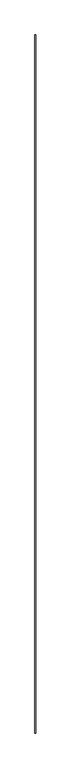
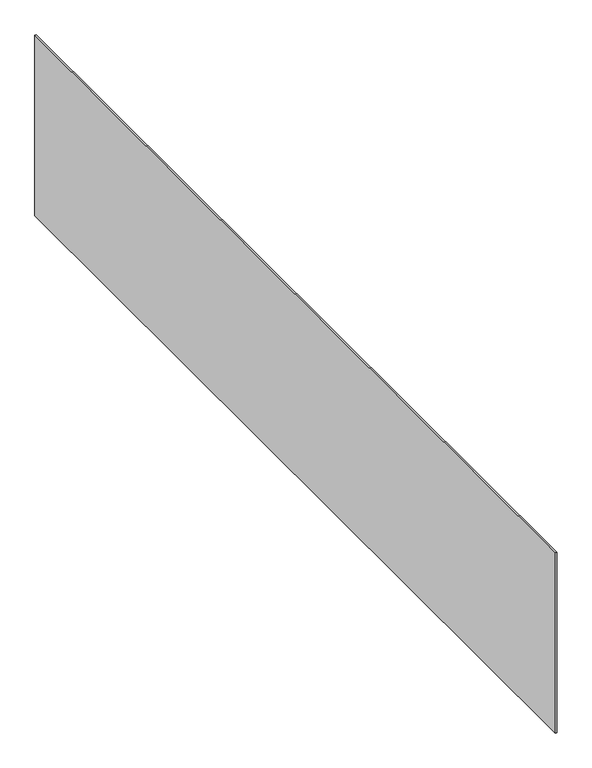
"""IFC4 building model written with IfcOpenShell, lengths in millimetres: proxy geometry, Panel:Panel:300402:Panel:300402 : Panel:Panel:300402:300124:Panel:300402:Panel:300402 : Panel:Panel:300402:300124 : Panel:Panel:300402:Panel:300402 : Panel:Panel:300402:300124:15 : Panel:Panel:300402:Panel:300402 : Panel:Panel:300402:300124:Panel:300402:Panel:300402 : Panel:Panel:300402:300124 : Panel:Panel:300402:Panel:300402 : Panel:Panel:300402:300124:300083."""

from ifc_helpers import new_model, si_unit, frame, origin, place, context, project, spatial, polyline, outline, extrude, source, transform, mapped, element, save


def generic_models_08288b9a(model_context):
    return source(origin(), model_context, "Body", "SweptSolid", [
        extrude(outline(polyline([(560289.4617238, -572944.1405465), (560289.4617238, -578718.1163841), (560281.5242239, -578718.1163841), (560281.5242239, -572944.1405465), (560289.4617238, -572944.1405465)])), frame((0.0, 0.0, 4946.65), z_axis=(0.0, 0.0, 1.0), x_axis=(1.0, 0.0, 0.0)), (0.0, 0.0, 1.0), 1219.2),
    ])


if __name__ == "__main__":
    model = new_model("IFC4")
    model_context = context("Model", 3, world=origin())
    ifc_project = project(units=[si_unit("LENGTHUNIT", "METRE", prefix="MILLI")], contexts=[model_context])
    site = spatial("IfcSite", under=ifc_project)
    building = spatial("IfcBuilding", under=site)
    placement = place(None, origin())
    generic_models_shape = generic_models_08288b9a(model_context)
    element("IfcBuildingElementProxy", 1, Name="Panel:Panel:300402:Panel:300402 : Panel:Panel:300402:300124:Panel:300402:Panel:300402 : Panel:Panel:300402:300124 : Panel:Panel:300402:Panel:300402 : Panel:Panel:300402:300124:15 : Panel:Panel:300402:Panel:300402 : Panel:Panel:300402:300124:Panel:300402:Panel:300402 : Panel:Panel:300402:300124 : Panel:Panel:300402:Panel:300402 : Panel:Panel:300402:300124:300083", ObjectType="Panel:Panel:300402:Panel:300402 : Panel:Panel:300402:300124:Panel:300402:Panel:300402 : Panel:Panel:300402:300124 : Panel:Panel:300402:Panel:300402 : Panel:Panel:300402:300124:15 : Panel:Panel:300402:Panel:300402 : Panel:Panel:300402:300124:Panel:300402:Panel:300402 : Panel:Panel:300402:300124 : Panel:Panel:300402:Panel:300402 : Panel:Panel:300402:300124:300083", at=placement, inside=building, context=model_context, shape_type="MappedRepresentation", body=[
        mapped(generic_models_shape, transform((0.0, 0.0, 0.0), x_axis=(1.0, 0.0, 0.0), y_axis=(0.0, 1.0, 0.0), z_axis=(0.0, 0.0, 1.0))),
    ])
    save(model, "model.ifc")

# Revit data of these elements
# Type "Panel:Panel:300402:Panel:300402 : Panel:Panel:300402:300124:Panel:300402:Panel:300402 : Panel:Panel:300402:300124 : Panel:Panel:300402:Panel:300402 : Panel:Panel:300402:300124:15 : Panel:Panel:300402:Panel:300402 : Panel:Panel:300402:300124:Panel:300402:Panel:300402 : Panel:Panel:300402:300124 : Panel:Panel:300402:Panel:300402 : Panel:Panel:300402:300124:300083"
#   NameOverride = "Panel:Panel:300402:Panel:300402 : Panel:Panel:300402:300124:Panel:300402:Panel:300402 : Panel:Panel:300402:300124 : Panel:Panel:300402:Panel:300402 : Panel:Panel:300402:300124:300083"
#   ObjectTypeOverride = "Panel:300402:Panel:300402 : Panel:Panel:300402:300124 : Panel:Panel:300402:Panel:300402 : Panel:Panel:300402:300124"
#   Reference = "Panel"
#   Tag = "300083"
# Element 1 (IfcBuildingElementProxy, "Panel:Panel:300402:Panel:300402 : Panel:Panel:300402:300124:Panel:300402:Panel:300402 : Panel:Panel:300402:300124 : Panel:Panel:300402:Panel:300402 : Panel:Panel:300402:300124:15 : Panel:Panel:300402:Panel:300402 : Panel:Panel:300402:300124:Panel:300402:Panel:300402 : Panel:Panel:300402:300124 : Panel:Panel:300402:Panel:300402 : Panel:Panel:300402:300124:300083")
#   Materials on its faces: "5/16\" PHENOLIC RESIN PANELS (CLASS A FLAME SPREAD) - EXPOSED FASTENERS"
# Materials
#   "5/16\" PHENOLIC RESIN PANELS (CLASS A FLAME SPREAD) - EXPOSED FASTENERS": class "Unassigned", colour RGB 64 64 64, transparency 0, Keynote = "M07420000.01", Cost = 0
